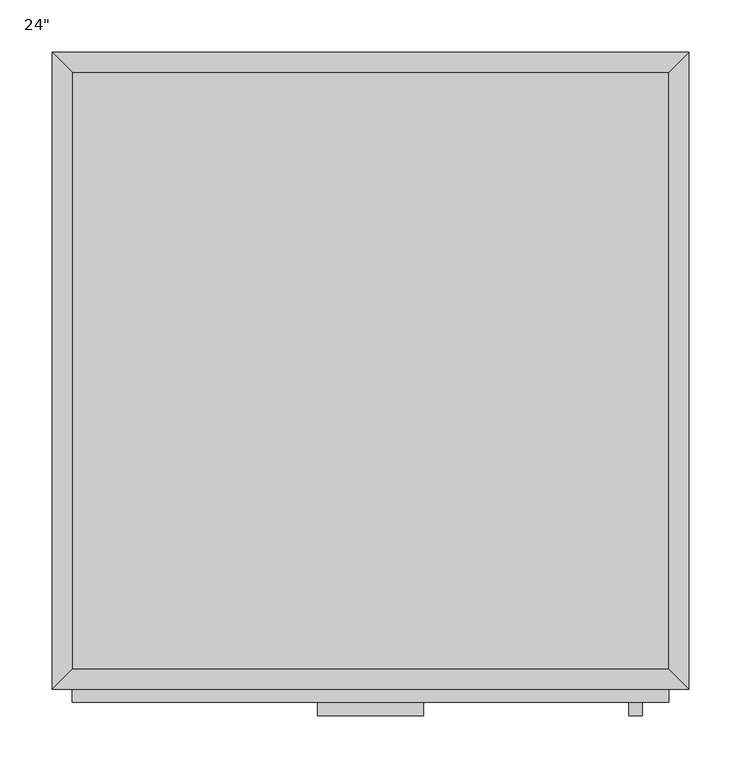
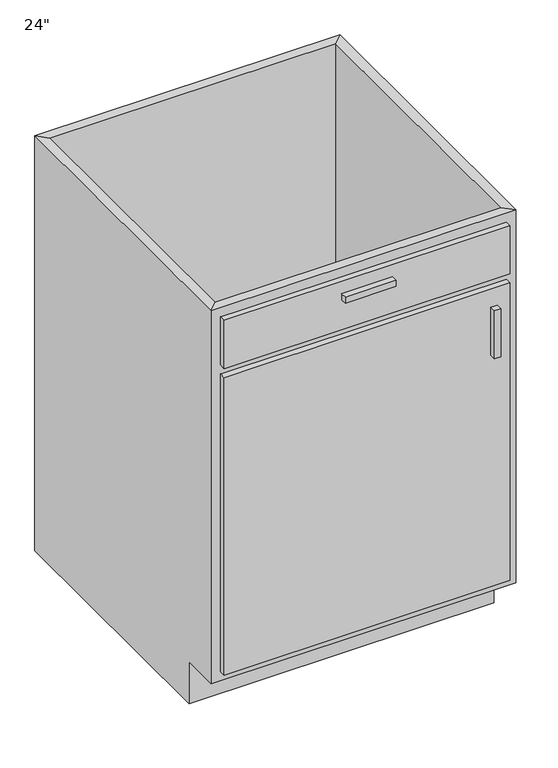
"""IFC4 building model written with IfcOpenShell, lengths in millimetres: furniture geometry."""

import ifcopenshell
import ifcopenshell.guid

model = None  # the IFC model being written
_history = None  # IfcOwnerHistory: only IFC2X3 demands one
_inside = {}  # id of a spatial element -> (the spatial element, [elements in it])
_under = {}  # id of a project, library or spatial element -> (it, [spatial elements below it])
_declared = {}  # id of a project -> (the project, [libraries it declares])
_typed = {}  # id of a type object -> (the type object, [elements of that type])
_made_of = {}  # id of a material, layer set ... -> (it, [elements and type objects made of it])


def new_model(schema):
    """Start an empty IFC model of exactly this schema.

    Asked for "IFC4X3", IfcOpenShell would pick the latest addendum, in which some entities
    have other attributes; the version numbers below select the first issue.
    IFC2X3 requires an IfcOwnerHistory on every rooted entity: one is made here for all.
    """
    global model, _history
    if schema == "IFC4X3":
        model = ifcopenshell.file(schema_version=(4, 3, 0, 0))
    else:
        model = ifcopenshell.file(schema=schema)
    _inside.clear()
    _under.clear()
    _declared.clear()
    _typed.clear()
    _made_of.clear()
    _history = None
    if model.schema == "IFC2X3":
        org = make("IfcOrganization", Name="unknown")
        user = make(
            "IfcPersonAndOrganization",
            ThePerson=make("IfcPerson", FamilyName="unknown"),
            TheOrganization=org,
        )
        app = make(
            "IfcApplication",
            ApplicationDeveloper=org,
            Version="unknown",
            ApplicationFullName="unknown",
            ApplicationIdentifier="unknown",
        )
        _history = make(
            "IfcOwnerHistory",
            OwningUser=user,
            OwningApplication=app,
            ChangeAction="ADDED",
            CreationDate=0,
        )
    return model


def make(cls, **values):
    """One entity of the class cls with the attributes given. An attribute that is None is left unset."""
    return model.create_entity(
        cls, **{name: value for name, value in values.items() if value is not None}
    )


def rooted(cls, **values):
    """An entity with a GlobalId (a new one), such as an element, a storey or a relation."""
    return make(cls, GlobalId=ifcopenshell.guid.new(), OwnerHistory=_history, **values)


def si_unit(unit_type, name, prefix=None):
    """IfcSIUnit, for example si_unit("LENGTHUNIT", "METRE", prefix="MILLI")."""
    return make("IfcSIUnit", UnitType=unit_type, Prefix=prefix, Name=name)


def assignment(units):
    """IfcUnitAssignment: the units of a project."""
    return None if units is None else make("IfcUnitAssignment", Units=units)


def point(xyz):
    """IfcCartesianPoint."""
    return None if xyz is None else make("IfcCartesianPoint", Coordinates=xyz)


def direction(xyz):
    """IfcDirection."""
    return None if xyz is None else make("IfcDirection", DirectionRatios=xyz)


def frame(location, z_axis=None, x_axis=None):
    """IfcAxis2Placement3D, a coordinate frame: its origin and axes. An axis left out is left unset."""
    return make(
        "IfcAxis2Placement3D",
        Location=point(location),
        Axis=direction(z_axis),
        RefDirection=direction(x_axis),
    )


def origin():
    """The frame at (0, 0, 0) with its axes left unset."""
    return frame((0.0, 0.0, 0.0))


def place(relative_to, where):
    """IfcLocalPlacement: puts the frame where relative to a parent placement (None: the world)."""
    return make(
        "IfcLocalPlacement", PlacementRelTo=relative_to, RelativePlacement=where
    )


def context(
    kind, dimensions, precision=None, world=None, true_north=None, identifier=None
):
    """IfcGeometricRepresentationContext, for example the 3D "Model" context."""
    return make(
        "IfcGeometricRepresentationContext",
        ContextIdentifier=identifier,
        ContextType=kind,
        CoordinateSpaceDimension=dimensions,
        Precision=precision,
        WorldCoordinateSystem=world,
        TrueNorth=true_north,
    )


def project(units=None, contexts=None):
    """IfcProject with its units and contexts."""
    return rooted(
        "IfcProject",
        Name="project",
        RepresentationContexts=contexts,
        UnitsInContext=assignment(units),
    )


def spatial(cls, under=None, at=None, **own):
    """A site, building, storey or space (cls), placed at a placement, below another one or the project."""
    s = rooted(cls, ObjectPlacement=at, **own)
    if under is not None:
        _under.setdefault(under.id(), (under, []))[1].append(s)
    return s


def polyline(points):
    """IfcPolyline through the points."""
    return make("IfcPolyline", Points=[point(p) for p in points])


def outline(outer, holes=None, kind="AREA"):
    """IfcArbitraryClosedProfileDef: a profile drawn as a closed curve; with holes, ...WithVoids."""
    if holes is None:
        return make("IfcArbitraryClosedProfileDef", ProfileType=kind, OuterCurve=outer)
    return make(
        "IfcArbitraryProfileDefWithVoids",
        ProfileType=kind,
        OuterCurve=outer,
        InnerCurves=holes,
    )


def extrude(swept, where, along, depth):
    """IfcExtrudedAreaSolid: the profile swept, set in the frame where, extruded along a direction by depth."""
    return make(
        "IfcExtrudedAreaSolid",
        SweptArea=swept,
        Position=where,
        ExtrudedDirection=direction(along),
        Depth=depth,
    )


def faces_of(points, faces, orient=None, outer=None):
    """IfcFace entities. A face is a list of loops; a loop is a list of indices into points, from 0.

    orient and outer hold one flag for each loop. By default every Orientation is true, the
    first loop of a face is its IfcFaceOuterBound and the others are IfcFaceBound.
    """
    made = []
    for i, loops in enumerate(faces):
        bounds = []
        for j, loop in enumerate(loops):
            is_outer = j == 0 if outer is None else outer[i][j]
            bounds.append(
                make(
                    "IfcFaceOuterBound" if is_outer else "IfcFaceBound",
                    Bound=make("IfcPolyLoop", Polygon=[points[k] for k in loop]),
                    Orientation=True if orient is None else orient[i][j],
                )
            )
        made.append(make("IfcFace", Bounds=bounds))
    return made


def faceted_brep(points, faces, orient=None, outer=None, voids=None):
    """IfcFacetedBrep: a solid bounded by flat faces; with voids (closed shells), ...WithVoids."""
    shared = [point(p) for p in points]
    hull = make("IfcClosedShell", CfsFaces=faces_of(shared, faces, orient, outer))
    if voids is None:
        return make("IfcFacetedBrep", Outer=hull)
    return make(
        "IfcFacetedBrepWithVoids",
        Outer=hull,
        Voids=[
            make(cls, CfsFaces=faces_of(shared, fs, o, b)) for cls, fs, o, b in voids
        ],
    )


def shape(context_of_items, identifier, shape_type, items):
    """IfcShapeRepresentation: the items that make up one representation, for example the "Body"."""
    return make(
        "IfcShapeRepresentation",
        ContextOfItems=context_of_items,
        RepresentationIdentifier=identifier,
        RepresentationType=shape_type,
        Items=items,
    )


def source(mapping_origin, context_of_items, identifier, shape_type, items):
    """IfcRepresentationMap: a shape defined once, which mapped items show again and again."""
    return make(
        "IfcRepresentationMap",
        MappingOrigin=mapping_origin,
        MappedRepresentation=shape(context_of_items, identifier, shape_type, items),
    )


def transform(
    local_origin,
    x_axis=None,
    y_axis=None,
    z_axis=None,
    scale=None,
    scale2=None,
    scale3=None,
    uniform=True,
):
    """IfcCartesianTransformationOperator3D, or its non-uniform kind. x_axis, y_axis, z_axis: its Axis1, 2, 3."""
    if uniform:
        return make(
            "IfcCartesianTransformationOperator3D",
            Axis1=direction(x_axis),
            Axis2=direction(y_axis),
            LocalOrigin=point(local_origin),
            Scale=scale,
            Axis3=direction(z_axis),
        )
    return make(
        "IfcCartesianTransformationOperator3DnonUniform",
        Axis1=direction(x_axis),
        Axis2=direction(y_axis),
        LocalOrigin=point(local_origin),
        Scale=scale,
        Axis3=direction(z_axis),
        Scale2=scale2,
        Scale3=scale3,
    )


def mapped(mapping_source, mapping_target):
    """IfcMappedItem: shows the shape of a source again, moved by a transform."""
    return make(
        "IfcMappedItem", MappingSource=mapping_source, MappingTarget=mapping_target
    )


def made_of(thing, what):
    """Note that an element or type object is made of a material, layer set ...; save() writes the relation."""
    if what is not None:
        _made_of.setdefault(what.id(), (what, []))[1].append(thing)
    return thing


def element(
    cls,
    number,
    at=None,
    inside=None,
    cuts=None,
    type_object=None,
    material=None,
    context=None,
    identifier="Body",
    shape_type=None,
    held_by="IfcProductDefinitionShape",
    body=None,
    shapes=None,
    **own,
):
    """One element of the class cls, such as IfcWall. Its Tag is "e" and its number.

    at: its placement. inside: the storey or other place that contains it. cuts: it is an
    opening in that element (IfcRelVoidsElement). A single representation is given by context,
    identifier, shape_type and body (its items); several are given by shapes. held_by: the class
    of the entity that holds the representations. save() writes the other relations.
    """
    e = rooted(cls, Tag="e%d" % number, ObjectPlacement=at, **own)
    if body is not None:
        shapes = [shape(context, identifier, shape_type, body)]
    if shapes is not None:
        e.Representation = make(held_by, Representations=shapes)
    if inside is not None:
        _inside.setdefault(inside.id(), (inside, []))[1].append(e)
    if cuts is not None:
        rooted(
            "IfcRelVoidsElement", RelatingBuildingElement=cuts, RelatedOpeningElement=e
        )
    if type_object is not None:
        _typed.setdefault(type_object.id(), (type_object, []))[1].append(e)
    return made_of(e, material)


def aggregate(whole, parts):
    """IfcRelAggregates: a whole, such as a stair, and the parts it consists of."""
    return rooted("IfcRelAggregates", RelatingObject=whole, RelatedObjects=parts)


def save(model, path):
    """Write the relations noted so far, then the file.

    IfcRelAggregates (storeys below a building ...), IfcRelContainedInSpatialStructure (elements
    in a storey), IfcRelDefinesByType, IfcRelAssociatesMaterial and IfcRelDeclares: one each for
    every whole, place, type object, material and project.
    """
    for whole, parts in _under.values():
        aggregate(whole, parts)
    for where, things in _inside.values():
        rooted(
            "IfcRelContainedInSpatialStructure",
            RelatedElements=things,
            RelatingStructure=where,
        )
    for kind, things in _typed.values():
        rooted("IfcRelDefinesByType", RelatedObjects=things, RelatingType=kind)
    for what, things in _made_of.values():
        rooted("IfcRelAssociatesMaterial", RelatedObjects=things, RelatingMaterial=what)
    for by, libraries in _declared.values():
        rooted("IfcRelDeclares", RelatingContext=by, RelatedDefinitions=libraries)
    model.write(path)


def furniture_6a014568(model_context):
    return source(origin(), model_context, "Body", "SolidModel", [
        faceted_brep([(304.4877049, -590.55, 876.3), (304.4877049, -590.55, 88.9), (-267.0122951, -590.55, 88.9), (-267.0122951, -590.55, 876.3), (-286.0622951, -609.6, 876.3), (323.5377049, -609.6, 876.3), (-286.0622951, -609.6, 88.9), (323.5377049, -609.6, 88.9), (-267.0122951, -533.4, 88.9), (-267.0122951, -19.05, 88.9), (-267.0122951, -19.05, 876.3), (-286.0622951, 0.0, 876.3), (-286.0622951, 0.0, 0.0), (-286.0622951, -533.4, 0.0), (-286.0622951, -533.4, 88.9), (304.4877049, -19.05, 88.9), (304.4877049, -19.05, 876.3), (323.5377049, 0.0, 876.3), (323.5377049, 0.0, 0.0), (304.4877049, -533.4, 88.9), (323.5377049, -533.4, 88.9), (323.5377049, -533.4, 0.0)], [[[0, 1, 2, 3]], [[0, 3, 4, 5]], [[5, 4, 6, 7]], [[2, 1, 7, 6]], [[3, 2, 8, 9, 10]], [[4, 3, 10, 11]], [[6, 4, 11, 12, 13, 14]], [[2, 6, 14, 8]], [[10, 9, 15, 16]], [[11, 10, 16, 17]], [[12, 11, 17, 18]], [[1, 0, 16, 15, 19]], [[0, 5, 17, 16]], [[5, 7, 20, 21, 18, 17]], [[7, 1, 19, 20]], [[8, 19, 15, 9]], [[18, 21, 13, 12]], [[13, 21, 20, 19, 8, 14]]]),
        extrude(outline(polyline([(279.0877049, -635.0), (266.3877049, -635.0), (266.3877049, -622.3), (279.0877049, -622.3), (279.0877049, -635.0)])), frame((0.0, 0.0, 596.9), z_axis=(0.0, 0.0, 1.0), x_axis=(1.0, 0.0, 0.0)), (0.0, 0.0, 1.0), 101.6),
        extrude(outline(polyline([(69.5377049, -635.0), (-32.0622951, -635.0), (-32.0622951, -622.3), (69.5377049, -622.3), (69.5377049, -635.0)])), frame((0.0, 0.0, 819.15), z_axis=(0.0, 0.0, 1.0), x_axis=(1.0, 0.0, 0.0)), (0.0, 0.0, 1.0), 12.7),
        extrude(outline(polyline([(304.4877049, -622.3), (-267.0122951, -622.3), (-267.0122951, -609.6), (304.4877049, -609.6), (304.4877049, -622.3)])), frame((0.0, 0.0, 107.95), z_axis=(0.0, 0.0, 1.0), x_axis=(1.0, 0.0, 0.0)), (0.0, 0.0, 1.0), 628.65),
        extrude(outline(polyline([(304.4877049, -622.3), (-267.0122951, -622.3), (-267.0122951, -609.6), (304.4877049, -609.6), (304.4877049, -622.3)])), frame((0.0, 0.0, 755.65), z_axis=(0.0, 0.0, 1.0), x_axis=(1.0, 0.0, 0.0)), (0.0, 0.0, 1.0), 101.6),
        extrude(outline(polyline([(304.4877049, -19.05), (304.4877049, -590.55), (-267.0122951, -590.55), (-267.0122951, -19.05), (304.4877049, -19.05)])), frame((0.0, 0.0, 88.9), z_axis=(0.0, 0.0, 1.0), x_axis=(1.0, 0.0, 0.0)), (0.0, 0.0, 1.0), 19.05),
    ])


if __name__ == "__main__":
    model = new_model("IFC4")
    model_context = context("Model", 3, world=origin())
    ifc_project = project(units=[si_unit("LENGTHUNIT", "METRE", prefix="MILLI")], contexts=[model_context])
    site = spatial("IfcSite", under=ifc_project)
    building = spatial("IfcBuilding", under=site)
    placement = place(None, origin())
    furniture_shape = furniture_6a014568(model_context)
    element("IfcFurniture", 1, ObjectType="Base Cabinet-Single Door & Drawer : 24\"", at=placement, inside=building, context=model_context, shape_type="MappedRepresentation", body=[
        mapped(furniture_shape, transform((0.0, 0.0, 0.0), x_axis=(1.0, 0.0, 0.0), y_axis=(0.0, 1.0, 0.0), z_axis=(0.0, 0.0, 1.0))),
    ])
    save(model, "model.ifc")

# Revit data of these elements
# Type "Base Cabinet-Single Door & Drawer : 24\""
#   Assembly Code = "C1030410"
#   Depth = 2' - 0"
#   Height = 2' - 10 1/2"
#   Toe Depth = 0' - 3"
#   Toe Height = 0' - 3 1/2"
#   Width = 2' - 0"
#   Cabinet Material = Cherry
#   Drawer Material = Cherry
#   Handle Material = Steel, Chrome Plated
#   Default Elevation = 0
# Element 1 (IfcFurniture, "Base Cabinet-Single Door & Drawer : 24\"")
#   Materials on its faces: "Cherry", "Steel, Chrome Plated", "Cabinets"
# Materials
#   "Cherry": class "Wood", colour RGB 157 77 38, transparency 0, Description = "Prunus Serotina", Cost = 0
#   "Steel, Chrome Plated": class "Metal", colour RGB 120 120 120, transparency 0, Description = "Chromiuim plated steel", Cost = 0
#   "Cabinets": class "Unassigned", colour RGB 249 249 249, transparency 0
